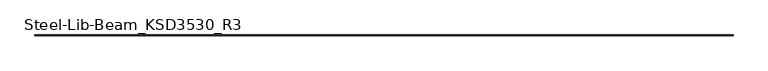
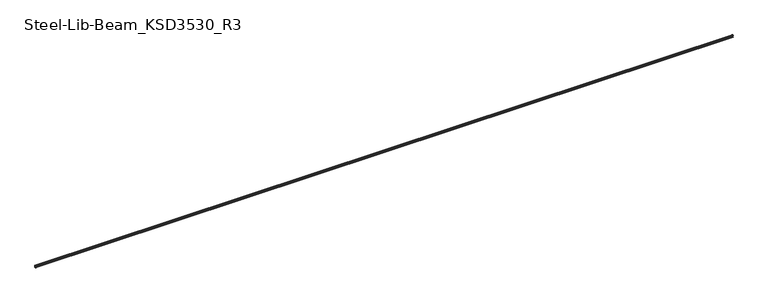
"""IFC4 building model written with IfcOpenShell, lengths in millimetres: beam geometry, Steel-Lib-Beam_KSD3530_R3 : BMS291_C-150×75x20x4.5."""

from ifc_helpers import new_model, si_unit, point, frame, frame_2d, origin, place, context, project, spatial, polyline, circle_curve, trimmed, segment, composite_curve, outline, extrude, source, transform, mapped, element, save


def steel_lib_beam_ksd3530_r3_ff58e29b(model_context):
    return source(origin(), model_context, "Body", "SweptSolid", [
        extrude(outline(composite_curve([segment(trimmed(circle_curve(frame_2d((-41.0, 66.0)), 9.0), [point((-50.0, 66.0))], [point((-41.0, 75.0))], False, "CARTESIAN"), True, "CONTINUOUS"), segment(polyline([(-41.0, 75.0), (16.0, 75.0)]), True, "CONTINUOUS"), segment(trimmed(circle_curve(frame_2d((16.0, 66.0)), 9.0), [point((16.0, 75.0))], [point((25.0, 66.0))], False, "CARTESIAN"), True, "CONTINUOUS"), segment(polyline([(25.0, 66.0), (25.0, -66.0)]), True, "CONTINUOUS"), segment(trimmed(circle_curve(frame_2d((16.0, -66.0)), 9.0), [point((25.0, -66.0))], [point((16.0, -75.0))], False, "CARTESIAN"), True, "CONTINUOUS"), segment(polyline([(16.0, -75.0), (-41.0, -75.0)]), True, "CONTINUOUS"), segment(trimmed(circle_curve(frame_2d((-41.0, -66.0)), 9.0), [point((-41.0, -75.0))], [point((-50.0, -66.0))], False, "CARTESIAN"), True, "CONTINUOUS"), segment(polyline([(-50.0, -66.0), (-50.0, -55.0), (-45.5, -55.0), (-45.5, -66.0)]), True, "CONTINUOUS"), segment(trimmed(circle_curve(frame_2d((-41.0, -66.0)), 4.5), [point((-45.5, -66.0))], [point((-41.0, -70.5))], True, "CARTESIAN"), True, "CONTINUOUS"), segment(polyline([(-41.0, -70.5), (16.0, -70.5)]), True, "CONTINUOUS"), segment(trimmed(circle_curve(frame_2d((16.0, -66.0)), 4.5), [point((16.0, -70.5))], [point((20.5, -66.0))], True, "CARTESIAN"), True, "CONTINUOUS"), segment(polyline([(20.5, -66.0), (20.5, 66.0)]), True, "CONTINUOUS"), segment(trimmed(circle_curve(frame_2d((16.0, 66.0)), 4.5), [point((20.5, 66.0))], [point((16.0, 70.5))], True, "CARTESIAN"), True, "CONTINUOUS"), segment(polyline([(16.0, 70.5), (-41.0, 70.5)]), True, "CONTINUOUS"), segment(trimmed(circle_curve(frame_2d((-41.0, 66.0)), 4.5), [point((-41.0, 70.5))], [point((-45.5, 66.0))], True, "CARTESIAN"), True, "CONTINUOUS"), segment(polyline([(-45.5, 66.0), (-45.5, 55.0), (-50.0, 55.0), (-50.0, 66.0)]), True, "CONTINUOUS")], self_intersect=False)), frame((-25654.5, 0.0, 0.0), z_axis=(1.0, 0.0, 0.0), x_axis=(0.0, 1.0, 0.0)), (0.0, 0.0, 1.0), 51309.0),
    ])


if __name__ == "__main__":
    model = new_model("IFC4")
    model_context = context("Model", 3, world=origin())
    ifc_project = project(units=[si_unit("LENGTHUNIT", "METRE", prefix="MILLI")], contexts=[model_context])
    site = spatial("IfcSite", under=ifc_project)
    building = spatial("IfcBuilding", under=site)
    placement = place(None, origin())
    steel_lib_beam_ksd3530_r3_shape = steel_lib_beam_ksd3530_r3_ff58e29b(model_context)
    element("IfcBeam", 1, ObjectType="Steel-Lib-Beam_KSD3530_R3 : BMS291_C-150×75x20x4.5", at=placement, inside=building, context=model_context, shape_type="MappedRepresentation", body=[
        mapped(steel_lib_beam_ksd3530_r3_shape, transform((0.0, 0.0, 0.0), x_axis=(1.0, 0.0, 0.0), y_axis=(0.0, 1.0, 0.0), z_axis=(0.0, 0.0, 1.0))),
    ])
    save(model, "model.ifc")

# Revit data of these elements
# Type "Steel-Lib-Beam_KSD3530_R3 : BMS291_C-150×75x20x4.5"
#   Keynote = "C-150×75x20x4.5"
#   SteelWeight = "Light"
#   x = 0.0250 m
#   t1 = 0.0090 m
#   t = 0.0045 m
#   Surface Area = 0.629834 m²/m
#   Section Area = 13.9688 cm²
#   Mass per Unit Length = 10.9655 kg/m
#   C = 0.0200 m
#   A = 0.0750 m
#   Length [instance default] = 1.5000 m
#   H = 0.1500 m
#   hec_material4 [instance default] = none
#   hec_material3 [instance default] = none
#   hec_material2 [instance default] = none
#   hec_material1 [instance default] = none
#   Structural Material [instance default] = Metal - Steel - Light Gauge
#   Assembly Code = ""
# Element 1 (IfcBeam, "Steel-Lib-Beam_KSD3530_R3 : BMS291_C-150×75x20x4.5")
#   Structural Material = none
# Materials
#   "Metal - Steel - Light Gauge": class "Metal", colour RGB 247 247 247, transparency 0
